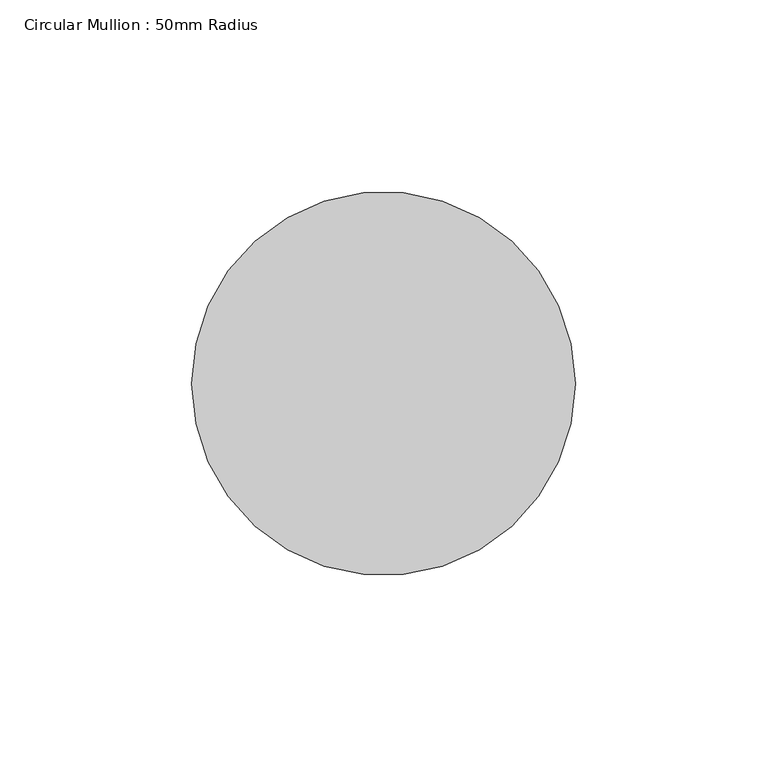
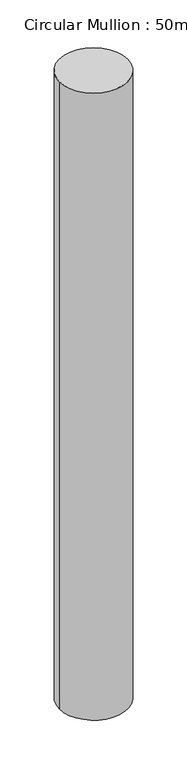
"""IFC4 building model written with IfcOpenShell, lengths in millimetres: member geometry, Circular Mullion : 50mm Radius."""

from ifc_helpers import new_model, si_unit, point, frame, origin, origin_2d, place, context, project, spatial, circle_curve, trimmed, segment, composite_curve, outline, extrude, source, transform, mapped, element, save


def circular_mullion_50mm_radius_0e9975d3(model_context):
    return source(origin(), model_context, "Body", "SweptSolid", [
        extrude(outline(composite_curve([segment(trimmed(circle_curve(origin_2d(), 50.0), [point((50.0, 0.0))], [point((-50.0, 0.0))], False, "CARTESIAN"), True, "CONTINUOUS"), segment(trimmed(circle_curve(origin_2d(), 50.0), [point((-50.0, 0.0))], [point((50.0, 0.0))], False, "CARTESIAN"), True, "CONTINUOUS")], self_intersect=False)), frame((0.0, 0.0, -969.4545001), z_axis=(0.0, 0.0, 1.0), x_axis=(1.0, 0.0, 0.0)), (0.0, 0.0, 1.0), 969.4545001),
    ])


if __name__ == "__main__":
    model = new_model("IFC4")
    model_context = context("Model", 3, world=origin())
    ifc_project = project(units=[si_unit("LENGTHUNIT", "METRE", prefix="MILLI")], contexts=[model_context])
    site = spatial("IfcSite", under=ifc_project)
    building = spatial("IfcBuilding", under=site)
    placement = place(None, origin())
    circular_mullion_50mm_radius_shape = circular_mullion_50mm_radius_0e9975d3(model_context)
    element("IfcMember", 1, ObjectType="Circular Mullion : 50mm Radius", at=placement, inside=building, context=model_context, shape_type="MappedRepresentation", body=[
        mapped(circular_mullion_50mm_radius_shape, transform((0.0, 0.0, 0.0), x_axis=(1.0, 0.0, 0.0), y_axis=(0.0, 1.0, 0.0), z_axis=(0.0, 0.0, 1.0))),
    ])
    save(model, "model.ifc")

# Revit data of these elements
# Type "Circular Mullion : 50mm Radius"
#   built-in parameter 1007350 = 0.164042 (stored number, unit not read)
# Element 1 (IfcMember, "Circular Mullion : 50mm Radius")
#   Materials on its faces: "Aluminium"
# Materials
#   "Aluminium": class "Metal", colour RGB 247 247 247, transparency 0, Description = "Aluminium 6061", Cost = 0
